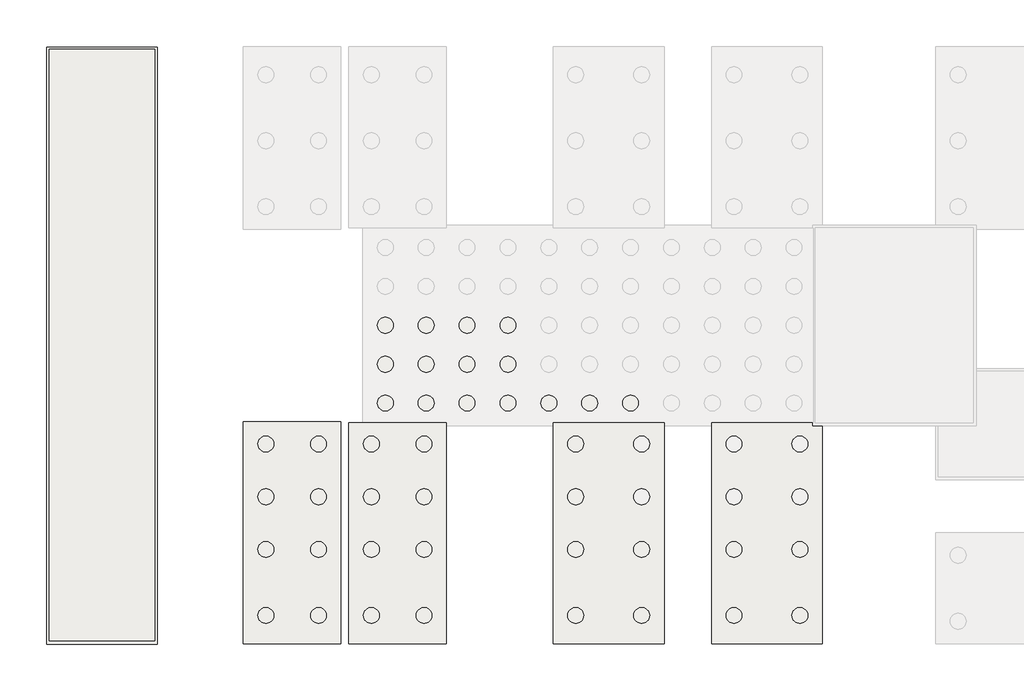
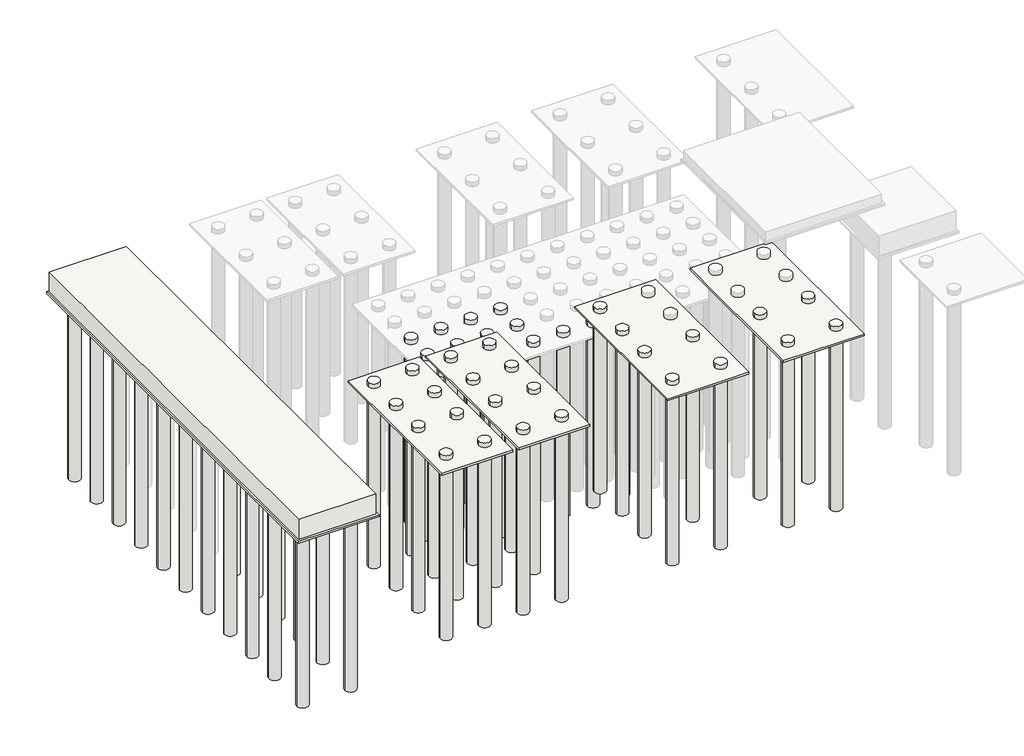
# One storey, part 1 of 3: 64 slabs.
"""IFC4 building model written with IfcOpenShell, lengths in millimetres."""

from ifc_helpers import new_model, si_unit, point, frame, frame_2d, origin, place, context, project, spatial, polyline, circle_curve, trimmed, segment, composite_curve, outline, extrude, faceted_brep, element, save

model = new_model("IFC4")

# Units and contexts
model_context = context("Model", 3, world=origin())
ifc_project = project(units=[si_unit("LENGTHUNIT", "METRE", prefix="MILLI")], contexts=[model_context])

# Site, building, storey
site = spatial("IfcSite", under=ifc_project)
building = spatial("IfcBuilding", under=site)
storey = spatial("IfcBuildingStorey", under=building, Name="B.O.F(FDN)", Elevation=-2500.0279945)

# Slabs
placement = place(None, origin())
element("IfcSlab", 1, ObjectType="H_SF_ACF_Lean_T100", at=placement, inside=storey, context=model_context, shape_type="SweptSolid", body=[
    extrude(outline(polyline([(1885.0, 41294.825326), (1885.0, 18654.825326), (-2315.0, 18654.825326), (-2315.0, 41294.825326), (1885.0, 41294.825326)])), frame((0.0, 0.0, -3699.3639791), z_axis=(0.0, 0.0, 1.0), x_axis=(1.0, 0.0, 0.0)), (0.0, 0.0, 1.0), 100.0),
])
element("IfcSlab", 2, ObjectType="H_SF_ACF_Lean_T100", at=placement, inside=storey, context=model_context, shape_type="SweptSolid", body=[
    extrude(outline(polyline([(8850.0, 27099.5208589), (8850.0, 18679.5208589), (5150.0, 18679.5208589), (5150.0, 27099.5208589), (8850.0, 27099.5208589)])), frame((0.0, 0.0, -2600.0279945), z_axis=(0.0, 0.0, 1.0), x_axis=(1.0, 0.0, 0.0)), (0.0, 0.0, 1.0), 100.0),
])
element("IfcSlab", 3, ObjectType="H_SF_ACF_Lean_T100", at=placement, inside=storey, context=model_context, shape_type="SweptSolid", body=[
    extrude(outline(polyline([(12850.0, 27049.5208589), (12850.0, 18679.5208589), (9150.0, 18679.5208589), (9150.0, 27049.5208589), (12850.0, 27049.5208589)])), frame((0.0, 0.0, -2600.0279945), z_axis=(0.0, 0.0, 1.0), x_axis=(1.0, 0.0, 0.0)), (0.0, 0.0, 1.0), 100.0),
])
element("IfcSlab", 4, ObjectType="H_SF_ACF_Lean_T100", at=placement, inside=storey, context=model_context, shape_type="SweptSolid", body=[
    extrude(outline(polyline([(21100.0, 18679.5208589), (16900.0, 18679.5208589), (16900.0, 27049.5208589), (21100.0, 27049.5208589), (21100.0, 18679.5208589)])), frame((0.0, 0.0, -2600.0279945), z_axis=(0.0, 0.0, 1.0), x_axis=(1.0, 0.0, 0.0)), (0.0, 0.0, 1.0), 100.0),
])
element("IfcSlab", 5, ObjectType="H_SF_ACF_Lean_T100", at=placement, inside=storey, context=model_context, shape_type="Brep", body=[
    faceted_brep([(27100.0, 18679.5208589, -2600.0279945), (22900.0, 18679.5208589, -2600.0279945), (22900.0, 27049.5208589, -2600.0279945), (27100.0, 27049.5208589, -2600.0279945), (27100.0, 18679.5208589, -2500.0279945), (27100.0, 27049.5208589, -2500.0279945), (26780.0, 27049.5208589, -2500.0279945), (26730.0, 27049.5208589, -2500.0279945), (22900.0, 27049.5208589, -2500.0279945), (22900.0, 18679.5208589, -2500.0279945)], [[[0, 1, 2, 3]], [[4, 5, 6, 7, 8, 9]], [[1, 0, 4, 9]], [[2, 1, 9, 8]], [[3, 2, 8, 7, 6, 5]], [[0, 3, 5, 4]]]),
])
element("IfcSlab", 6, ObjectType="Foundation Rectangular(Non-Pile) : H_SF_ACF_W4000xL22440xT1100_Protection", at=placement, inside=storey, context=model_context, shape_type="SweptSolid", body=[
    extrude(outline(polyline([(-2215.0, 41219.5208589), (1785.0, 41219.5208589), (1785.0, 18779.5208589), (-2215.0, 18779.5208589), (-2215.0, 41219.5208589)])), frame((0.0, 0.0, -3599.3639791), z_axis=(0.0, 0.0, 1.0), x_axis=(1.0, 0.0, 0.0)), (0.0, 0.0, 1.0), 1099.3359846),
])
element("IfcSlab", 7, ObjectType="Pile : H_SF_API_Steel Pile D508x12t_L10m", at=placement, inside=storey, context=model_context, shape_type="SweptSolid", body=[
    extrude(outline(composite_curve([segment(trimmed(circle_curve(frame_2d((-1465.0, 40249.5208589)), 300.0), [point((-1765.0, 40249.5208589))], [point((-1165.0, 40249.5208589))], False, "CARTESIAN"), True, "CONTINUOUS"), segment(trimmed(circle_curve(frame_2d((-1465.0, 40249.5208589)), 300.0), [point((-1165.0, 40249.5208589))], [point((-1765.0, 40249.5208589))], False, "CARTESIAN"), True, "CONTINUOUS")], self_intersect=False)), frame((0.0, 0.0, -13500.0279945), z_axis=(0.0, 0.0, 1.0), x_axis=(1.0, 0.0, 0.0)), (0.0, 0.0, 1.0), 10150.0),
])
element("IfcSlab", 8, ObjectType="Pile : H_SF_API_Steel Pile D508x12t_L10m", at=placement, inside=storey, context=model_context, shape_type="SweptSolid", body=[
    extrude(outline(composite_curve([segment(trimmed(circle_curve(frame_2d((-1465.0, 19749.5208589)), 300.0), [point((-1765.0, 19749.5208589))], [point((-1165.0, 19749.5208589))], False, "CARTESIAN"), True, "CONTINUOUS"), segment(trimmed(circle_curve(frame_2d((-1465.0, 19749.5208589)), 300.0), [point((-1165.0, 19749.5208589))], [point((-1765.0, 19749.5208589))], False, "CARTESIAN"), True, "CONTINUOUS")], self_intersect=False)), frame((0.0, 0.0, -13500.0279945), z_axis=(0.0, 0.0, 1.0), x_axis=(1.0, 0.0, 0.0)), (0.0, 0.0, 1.0), 10150.0),
])
element("IfcSlab", 9, ObjectType="Pile : H_SF_API_Steel Pile D508x12t_L10m", at=placement, inside=storey, context=model_context, shape_type="SweptSolid", body=[
    extrude(outline(composite_curve([segment(trimmed(circle_curve(frame_2d((1035.0, 19749.5208589)), 300.0), [point((1335.0, 19749.5208589))], [point((735.0, 19749.5208589))], False, "CARTESIAN"), True, "CONTINUOUS"), segment(trimmed(circle_curve(frame_2d((1035.0, 19749.5208589)), 300.0), [point((735.0, 19749.5208589))], [point((1335.0, 19749.5208589))], False, "CARTESIAN"), True, "CONTINUOUS")], self_intersect=False)), frame((0.0, 0.0, -13500.0279945), z_axis=(0.0, 0.0, 1.0), x_axis=(1.0, 0.0, 0.0)), (0.0, 0.0, 1.0), 10150.0),
])
element("IfcSlab", 10, ObjectType="Pile : H_SF_API_Steel Pile D508x12t_L10m", at=placement, inside=storey, context=model_context, shape_type="SweptSolid", body=[
    extrude(outline(composite_curve([segment(trimmed(circle_curve(frame_2d((-1465.0, 38249.5208589)), 300.0), [point((-1765.0, 38249.5208589))], [point((-1165.0, 38249.5208589))], False, "CARTESIAN"), True, "CONTINUOUS"), segment(trimmed(circle_curve(frame_2d((-1465.0, 38249.5208589)), 300.0), [point((-1165.0, 38249.5208589))], [point((-1765.0, 38249.5208589))], False, "CARTESIAN"), True, "CONTINUOUS")], self_intersect=False)), frame((0.0, 0.0, -13500.0279945), z_axis=(0.0, 0.0, 1.0), x_axis=(1.0, 0.0, 0.0)), (0.0, 0.0, 1.0), 10150.0),
])
element("IfcSlab", 11, ObjectType="Pile : H_SF_API_Steel Pile D508x12t_L10m", at=placement, inside=storey, context=model_context, shape_type="SweptSolid", body=[
    extrude(outline(composite_curve([segment(trimmed(circle_curve(frame_2d((-1465.0, 36249.5208589)), 300.0), [point((-1765.0, 36249.5208589))], [point((-1165.0, 36249.5208589))], False, "CARTESIAN"), True, "CONTINUOUS"), segment(trimmed(circle_curve(frame_2d((-1465.0, 36249.5208589)), 300.0), [point((-1165.0, 36249.5208589))], [point((-1765.0, 36249.5208589))], False, "CARTESIAN"), True, "CONTINUOUS")], self_intersect=False)), frame((0.0, 0.0, -13500.0279945), z_axis=(0.0, 0.0, 1.0), x_axis=(1.0, 0.0, 0.0)), (0.0, 0.0, 1.0), 10150.0),
])
element("IfcSlab", 12, ObjectType="Pile : H_SF_API_Steel Pile D508x12t_L10m", at=placement, inside=storey, context=model_context, shape_type="SweptSolid", body=[
    extrude(outline(composite_curve([segment(trimmed(circle_curve(frame_2d((-1465.0, 34249.5208589)), 300.0), [point((-1765.0, 34249.5208589))], [point((-1165.0, 34249.5208589))], False, "CARTESIAN"), True, "CONTINUOUS"), segment(trimmed(circle_curve(frame_2d((-1465.0, 34249.5208589)), 300.0), [point((-1165.0, 34249.5208589))], [point((-1765.0, 34249.5208589))], False, "CARTESIAN"), True, "CONTINUOUS")], self_intersect=False)), frame((0.0, 0.0, -13500.0279945), z_axis=(0.0, 0.0, 1.0), x_axis=(1.0, 0.0, 0.0)), (0.0, 0.0, 1.0), 10150.0),
])
element("IfcSlab", 13, ObjectType="Pile : H_SF_API_Steel Pile D508x12t_L10m", at=placement, inside=storey, context=model_context, shape_type="SweptSolid", body=[
    extrude(outline(composite_curve([segment(trimmed(circle_curve(frame_2d((-1465.0, 32249.5208589)), 300.0), [point((-1765.0, 32249.5208589))], [point((-1165.0, 32249.5208589))], False, "CARTESIAN"), True, "CONTINUOUS"), segment(trimmed(circle_curve(frame_2d((-1465.0, 32249.5208589)), 300.0), [point((-1165.0, 32249.5208589))], [point((-1765.0, 32249.5208589))], False, "CARTESIAN"), True, "CONTINUOUS")], self_intersect=False)), frame((0.0, 0.0, -13500.0279945), z_axis=(0.0, 0.0, 1.0), x_axis=(1.0, 0.0, 0.0)), (0.0, 0.0, 1.0), 10150.0),
])
element("IfcSlab", 14, ObjectType="Pile : H_SF_API_Steel Pile D508x12t_L10m", at=placement, inside=storey, context=model_context, shape_type="SweptSolid", body=[
    extrude(outline(composite_curve([segment(trimmed(circle_curve(frame_2d((-1465.0, 30249.5208589)), 300.0), [point((-1765.0, 30249.5208589))], [point((-1165.0, 30249.5208589))], False, "CARTESIAN"), True, "CONTINUOUS"), segment(trimmed(circle_curve(frame_2d((-1465.0, 30249.5208589)), 300.0), [point((-1165.0, 30249.5208589))], [point((-1765.0, 30249.5208589))], False, "CARTESIAN"), True, "CONTINUOUS")], self_intersect=False)), frame((0.0, 0.0, -13500.0279945), z_axis=(0.0, 0.0, 1.0), x_axis=(1.0, 0.0, 0.0)), (0.0, 0.0, 1.0), 10150.0),
])
element("IfcSlab", 15, ObjectType="Pile : H_SF_API_Steel Pile D508x12t_L10m", at=placement, inside=storey, context=model_context, shape_type="SweptSolid", body=[
    extrude(outline(composite_curve([segment(trimmed(circle_curve(frame_2d((1035.0, 30249.5208589)), 300.0), [point((1335.0, 30249.5208589))], [point((735.0, 30249.5208589))], False, "CARTESIAN"), True, "CONTINUOUS"), segment(trimmed(circle_curve(frame_2d((1035.0, 30249.5208589)), 300.0), [point((735.0, 30249.5208589))], [point((1335.0, 30249.5208589))], False, "CARTESIAN"), True, "CONTINUOUS")], self_intersect=False)), frame((0.0, 0.0, -13500.0279945), z_axis=(0.0, 0.0, 1.0), x_axis=(1.0, 0.0, 0.0)), (0.0, 0.0, 1.0), 10150.0),
])
element("IfcSlab", 16, ObjectType="Pile : H_SF_API_Steel Pile D508x12t_L10m", at=placement, inside=storey, context=model_context, shape_type="SweptSolid", body=[
    extrude(outline(composite_curve([segment(trimmed(circle_curve(frame_2d((-1465.0, 28249.5208589)), 300.0), [point((-1765.0, 28249.5208589))], [point((-1165.0, 28249.5208589))], False, "CARTESIAN"), True, "CONTINUOUS"), segment(trimmed(circle_curve(frame_2d((-1465.0, 28249.5208589)), 300.0), [point((-1165.0, 28249.5208589))], [point((-1765.0, 28249.5208589))], False, "CARTESIAN"), True, "CONTINUOUS")], self_intersect=False)), frame((0.0, 0.0, -13500.0279945), z_axis=(0.0, 0.0, 1.0), x_axis=(1.0, 0.0, 0.0)), (0.0, 0.0, 1.0), 10150.0),
])
element("IfcSlab", 17, ObjectType="Pile : H_SF_API_Steel Pile D508x12t_L10m", at=placement, inside=storey, context=model_context, shape_type="SweptSolid", body=[
    extrude(outline(composite_curve([segment(trimmed(circle_curve(frame_2d((1035.0, 28249.5208589)), 300.0), [point((1335.0, 28249.5208589))], [point((735.0, 28249.5208589))], False, "CARTESIAN"), True, "CONTINUOUS"), segment(trimmed(circle_curve(frame_2d((1035.0, 28249.5208589)), 300.0), [point((735.0, 28249.5208589))], [point((1335.0, 28249.5208589))], False, "CARTESIAN"), True, "CONTINUOUS")], self_intersect=False)), frame((0.0, 0.0, -13500.0279945), z_axis=(0.0, 0.0, 1.0), x_axis=(1.0, 0.0, 0.0)), (0.0, 0.0, 1.0), 10150.0),
])
element("IfcSlab", 18, ObjectType="Pile : H_SF_API_Steel Pile D508x12t_L10m", at=placement, inside=storey, context=model_context, shape_type="SweptSolid", body=[
    extrude(outline(composite_curve([segment(trimmed(circle_curve(frame_2d((-1465.0, 26249.5208589)), 300.0), [point((-1765.0, 26249.5208589))], [point((-1165.0, 26249.5208589))], False, "CARTESIAN"), True, "CONTINUOUS"), segment(trimmed(circle_curve(frame_2d((-1465.0, 26249.5208589)), 300.0), [point((-1165.0, 26249.5208589))], [point((-1765.0, 26249.5208589))], False, "CARTESIAN"), True, "CONTINUOUS")], self_intersect=False)), frame((0.0, 0.0, -13500.0279945), z_axis=(0.0, 0.0, 1.0), x_axis=(1.0, 0.0, 0.0)), (0.0, 0.0, 1.0), 10150.0),
])
element("IfcSlab", 19, ObjectType="Pile : H_SF_API_Steel Pile D508x12t_L10m", at=placement, inside=storey, context=model_context, shape_type="SweptSolid", body=[
    extrude(outline(composite_curve([segment(trimmed(circle_curve(frame_2d((1035.0, 26249.5208589)), 300.0), [point((1335.0, 26249.5208589))], [point((735.0, 26249.5208589))], False, "CARTESIAN"), True, "CONTINUOUS"), segment(trimmed(circle_curve(frame_2d((1035.0, 26249.5208589)), 300.0), [point((735.0, 26249.5208589))], [point((1335.0, 26249.5208589))], False, "CARTESIAN"), True, "CONTINUOUS")], self_intersect=False)), frame((0.0, 0.0, -13500.0279945), z_axis=(0.0, 0.0, 1.0), x_axis=(1.0, 0.0, 0.0)), (0.0, 0.0, 1.0), 10150.0),
])
element("IfcSlab", 20, ObjectType="Pile : H_SF_API_Steel Pile D508x12t_L10m", at=placement, inside=storey, context=model_context, shape_type="SweptSolid", body=[
    extrude(outline(composite_curve([segment(trimmed(circle_curve(frame_2d((-1465.0, 24249.5208589)), 300.0), [point((-1765.0, 24249.5208589))], [point((-1165.0, 24249.5208589))], False, "CARTESIAN"), True, "CONTINUOUS"), segment(trimmed(circle_curve(frame_2d((-1465.0, 24249.5208589)), 300.0), [point((-1165.0, 24249.5208589))], [point((-1765.0, 24249.5208589))], False, "CARTESIAN"), True, "CONTINUOUS")], self_intersect=False)), frame((0.0, 0.0, -13500.0279945), z_axis=(0.0, 0.0, 1.0), x_axis=(1.0, 0.0, 0.0)), (0.0, 0.0, 1.0), 10150.0),
])
element("IfcSlab", 21, ObjectType="Pile : H_SF_API_Steel Pile D508x12t_L10m", at=placement, inside=storey, context=model_context, shape_type="SweptSolid", body=[
    extrude(outline(composite_curve([segment(trimmed(circle_curve(frame_2d((1035.0, 24249.5208589)), 300.0), [point((1335.0, 24249.5208589))], [point((735.0, 24249.5208589))], False, "CARTESIAN"), True, "CONTINUOUS"), segment(trimmed(circle_curve(frame_2d((1035.0, 24249.5208589)), 300.0), [point((735.0, 24249.5208589))], [point((1335.0, 24249.5208589))], False, "CARTESIAN"), True, "CONTINUOUS")], self_intersect=False)), frame((0.0, 0.0, -13500.0279945), z_axis=(0.0, 0.0, 1.0), x_axis=(1.0, 0.0, 0.0)), (0.0, 0.0, 1.0), 10150.0),
])
element("IfcSlab", 22, ObjectType="Pile : H_SF_API_Steel Pile D508x12t_L10m", at=placement, inside=storey, context=model_context, shape_type="SweptSolid", body=[
    extrude(outline(composite_curve([segment(trimmed(circle_curve(frame_2d((-1465.0, 22249.5208589)), 300.0), [point((-1765.0, 22249.5208589))], [point((-1165.0, 22249.5208589))], False, "CARTESIAN"), True, "CONTINUOUS"), segment(trimmed(circle_curve(frame_2d((-1465.0, 22249.5208589)), 300.0), [point((-1165.0, 22249.5208589))], [point((-1765.0, 22249.5208589))], False, "CARTESIAN"), True, "CONTINUOUS")], self_intersect=False)), frame((0.0, 0.0, -13500.0279945), z_axis=(0.0, 0.0, 1.0), x_axis=(1.0, 0.0, 0.0)), (0.0, 0.0, 1.0), 10150.0),
])
element("IfcSlab", 23, ObjectType="Pile : H_SF_API_Steel Pile D508x12t_L10m", at=placement, inside=storey, context=model_context, shape_type="SweptSolid", body=[
    extrude(outline(composite_curve([segment(trimmed(circle_curve(frame_2d((1035.0, 22249.5208589)), 300.0), [point((1335.0, 22249.5208589))], [point((735.0, 22249.5208589))], False, "CARTESIAN"), True, "CONTINUOUS"), segment(trimmed(circle_curve(frame_2d((1035.0, 22249.5208589)), 300.0), [point((735.0, 22249.5208589))], [point((1335.0, 22249.5208589))], False, "CARTESIAN"), True, "CONTINUOUS")], self_intersect=False)), frame((0.0, 0.0, -13500.0279945), z_axis=(0.0, 0.0, 1.0), x_axis=(1.0, 0.0, 0.0)), (0.0, 0.0, 1.0), 10150.0),
])
element("IfcSlab", 24, ObjectType="Pile : H_SF_API_Steel Pile D508x12t_L10m", at=placement, inside=storey, context=model_context, shape_type="SweptSolid", body=[
    extrude(outline(composite_curve([segment(trimmed(circle_curve(frame_2d((8000.0, 19749.5208589)), 300.0), [point((8300.0, 19749.5208589))], [point((7700.0, 19749.5208589))], False, "CARTESIAN"), True, "CONTINUOUS"), segment(trimmed(circle_curve(frame_2d((8000.0, 19749.5208589)), 300.0), [point((7700.0, 19749.5208589))], [point((8300.0, 19749.5208589))], False, "CARTESIAN"), True, "CONTINUOUS")], self_intersect=False)), frame((0.0, 0.0, -12400.0279945), z_axis=(0.0, 0.0, 1.0), x_axis=(1.0, 0.0, 0.0)), (0.0, 0.0, 1.0), 10150.0),
])
element("IfcSlab", 25, ObjectType="Pile : H_SF_API_Steel Pile D508x12t_L10m", at=placement, inside=storey, context=model_context, shape_type="SweptSolid", body=[
    extrude(outline(composite_curve([segment(trimmed(circle_curve(frame_2d((6000.0, 19749.5208589)), 300.0), [point((5700.0, 19749.5208589))], [point((6300.0, 19749.5208589))], False, "CARTESIAN"), True, "CONTINUOUS"), segment(trimmed(circle_curve(frame_2d((6000.0, 19749.5208589)), 300.0), [point((6300.0, 19749.5208589))], [point((5700.0, 19749.5208589))], False, "CARTESIAN"), True, "CONTINUOUS")], self_intersect=False)), frame((0.0, 0.0, -12400.0279945), z_axis=(0.0, 0.0, 1.0), x_axis=(1.0, 0.0, 0.0)), (0.0, 0.0, 1.0), 10150.0),
])
element("IfcSlab", 26, ObjectType="Pile : H_SF_API_Steel Pile D508x12t_L10m", at=placement, inside=storey, context=model_context, shape_type="SweptSolid", body=[
    extrude(outline(composite_curve([segment(trimmed(circle_curve(frame_2d((8000.0, 22249.5208589)), 300.0), [point((8300.0, 22249.5208589))], [point((7700.0, 22249.5208589))], False, "CARTESIAN"), True, "CONTINUOUS"), segment(trimmed(circle_curve(frame_2d((8000.0, 22249.5208589)), 300.0), [point((7700.0, 22249.5208589))], [point((8300.0, 22249.5208589))], False, "CARTESIAN"), True, "CONTINUOUS")], self_intersect=False)), frame((0.0, 0.0, -12400.0279945), z_axis=(0.0, 0.0, 1.0), x_axis=(1.0, 0.0, 0.0)), (0.0, 0.0, 1.0), 10150.0),
])
element("IfcSlab", 27, ObjectType="Pile : H_SF_API_Steel Pile D508x12t_L10m", at=placement, inside=storey, context=model_context, shape_type="SweptSolid", body=[
    extrude(outline(composite_curve([segment(trimmed(circle_curve(frame_2d((6000.0, 22249.5208589)), 300.0), [point((5700.0, 22249.5208589))], [point((6300.0, 22249.5208589))], False, "CARTESIAN"), True, "CONTINUOUS"), segment(trimmed(circle_curve(frame_2d((6000.0, 22249.5208589)), 300.0), [point((6300.0, 22249.5208589))], [point((5700.0, 22249.5208589))], False, "CARTESIAN"), True, "CONTINUOUS")], self_intersect=False)), frame((0.0, 0.0, -12400.0279945), z_axis=(0.0, 0.0, 1.0), x_axis=(1.0, 0.0, 0.0)), (0.0, 0.0, 1.0), 10150.0),
])
element("IfcSlab", 28, ObjectType="Pile : H_SF_API_Steel Pile D508x12t_L10m", at=placement, inside=storey, context=model_context, shape_type="SweptSolid", body=[
    extrude(outline(composite_curve([segment(trimmed(circle_curve(frame_2d((8000.0, 24249.5208589)), 300.0), [point((8300.0, 24249.5208589))], [point((7700.0, 24249.5208589))], False, "CARTESIAN"), True, "CONTINUOUS"), segment(trimmed(circle_curve(frame_2d((8000.0, 24249.5208589)), 300.0), [point((7700.0, 24249.5208589))], [point((8300.0, 24249.5208589))], False, "CARTESIAN"), True, "CONTINUOUS")], self_intersect=False)), frame((0.0, 0.0, -12400.0279945), z_axis=(0.0, 0.0, 1.0), x_axis=(1.0, 0.0, 0.0)), (0.0, 0.0, 1.0), 10150.0),
])
element("IfcSlab", 29, ObjectType="Pile : H_SF_API_Steel Pile D508x12t_L10m", at=placement, inside=storey, context=model_context, shape_type="SweptSolid", body=[
    extrude(outline(composite_curve([segment(trimmed(circle_curve(frame_2d((6000.0, 24249.5208589)), 300.0), [point((5700.0, 24249.5208589))], [point((6300.0, 24249.5208589))], False, "CARTESIAN"), True, "CONTINUOUS"), segment(trimmed(circle_curve(frame_2d((6000.0, 24249.5208589)), 300.0), [point((6300.0, 24249.5208589))], [point((5700.0, 24249.5208589))], False, "CARTESIAN"), True, "CONTINUOUS")], self_intersect=False)), frame((0.0, 0.0, -12400.0279945), z_axis=(0.0, 0.0, 1.0), x_axis=(1.0, 0.0, 0.0)), (0.0, 0.0, 1.0), 10150.0),
])
element("IfcSlab", 30, ObjectType="Pile : H_SF_API_Steel Pile D508x12t_L10m", at=placement, inside=storey, context=model_context, shape_type="SweptSolid", body=[
    extrude(outline(composite_curve([segment(trimmed(circle_curve(frame_2d((8000.0, 26249.5208589)), 300.0), [point((8300.0, 26249.5208589))], [point((7700.0, 26249.5208589))], False, "CARTESIAN"), True, "CONTINUOUS"), segment(trimmed(circle_curve(frame_2d((8000.0, 26249.5208589)), 300.0), [point((7700.0, 26249.5208589))], [point((8300.0, 26249.5208589))], False, "CARTESIAN"), True, "CONTINUOUS")], self_intersect=False)), frame((0.0, 0.0, -12400.0279945), z_axis=(0.0, 0.0, 1.0), x_axis=(1.0, 0.0, 0.0)), (0.0, 0.0, 1.0), 10150.0),
])
element("IfcSlab", 31, ObjectType="Pile : H_SF_API_Steel Pile D508x12t_L10m", at=placement, inside=storey, context=model_context, shape_type="SweptSolid", body=[
    extrude(outline(composite_curve([segment(trimmed(circle_curve(frame_2d((6000.0, 26249.5208589)), 300.0), [point((5700.0, 26249.5208589))], [point((6300.0, 26249.5208589))], False, "CARTESIAN"), True, "CONTINUOUS"), segment(trimmed(circle_curve(frame_2d((6000.0, 26249.5208589)), 300.0), [point((6300.0, 26249.5208589))], [point((5700.0, 26249.5208589))], False, "CARTESIAN"), True, "CONTINUOUS")], self_intersect=False)), frame((0.0, 0.0, -12400.0279945), z_axis=(0.0, 0.0, 1.0), x_axis=(1.0, 0.0, 0.0)), (0.0, 0.0, 1.0), 10150.0),
])
element("IfcSlab", 32, ObjectType="Pile : H_SF_API_Steel Pile D508x12t_L10m", at=placement, inside=storey, context=model_context, shape_type="SweptSolid", body=[
    extrude(outline(composite_curve([segment(trimmed(circle_curve(frame_2d((12000.0, 19749.5208589)), 300.0), [point((12300.0, 19749.5208589))], [point((11700.0, 19749.5208589))], False, "CARTESIAN"), True, "CONTINUOUS"), segment(trimmed(circle_curve(frame_2d((12000.0, 19749.5208589)), 300.0), [point((11700.0, 19749.5208589))], [point((12300.0, 19749.5208589))], False, "CARTESIAN"), True, "CONTINUOUS")], self_intersect=False)), frame((0.0, 0.0, -12400.0279945), z_axis=(0.0, 0.0, 1.0), x_axis=(1.0, 0.0, 0.0)), (0.0, 0.0, 1.0), 10150.0),
])
element("IfcSlab", 33, ObjectType="Pile : H_SF_API_Steel Pile D508x12t_L10m", at=placement, inside=storey, context=model_context, shape_type="SweptSolid", body=[
    extrude(outline(composite_curve([segment(trimmed(circle_curve(frame_2d((10000.0, 19749.5208589)), 300.0), [point((9700.0, 19749.5208589))], [point((10300.0, 19749.5208589))], False, "CARTESIAN"), True, "CONTINUOUS"), segment(trimmed(circle_curve(frame_2d((10000.0, 19749.5208589)), 300.0), [point((10300.0, 19749.5208589))], [point((9700.0, 19749.5208589))], False, "CARTESIAN"), True, "CONTINUOUS")], self_intersect=False)), frame((0.0, 0.0, -12400.0279945), z_axis=(0.0, 0.0, 1.0), x_axis=(1.0, 0.0, 0.0)), (0.0, 0.0, 1.0), 10150.0),
])
element("IfcSlab", 34, ObjectType="Pile : H_SF_API_Steel Pile D508x12t_L10m", at=placement, inside=storey, context=model_context, shape_type="SweptSolid", body=[
    extrude(outline(composite_curve([segment(trimmed(circle_curve(frame_2d((12000.0, 22249.5208589)), 300.0), [point((12300.0, 22249.5208589))], [point((11700.0, 22249.5208589))], False, "CARTESIAN"), True, "CONTINUOUS"), segment(trimmed(circle_curve(frame_2d((12000.0, 22249.5208589)), 300.0), [point((11700.0, 22249.5208589))], [point((12300.0, 22249.5208589))], False, "CARTESIAN"), True, "CONTINUOUS")], self_intersect=False)), frame((0.0, 0.0, -12400.0279945), z_axis=(0.0, 0.0, 1.0), x_axis=(1.0, 0.0, 0.0)), (0.0, 0.0, 1.0), 10150.0),
])
element("IfcSlab", 35, ObjectType="Pile : H_SF_API_Steel Pile D508x12t_L10m", at=placement, inside=storey, context=model_context, shape_type="SweptSolid", body=[
    extrude(outline(composite_curve([segment(trimmed(circle_curve(frame_2d((10000.0, 22249.5208589)), 300.0), [point((9700.0, 22249.5208589))], [point((10300.0, 22249.5208589))], False, "CARTESIAN"), True, "CONTINUOUS"), segment(trimmed(circle_curve(frame_2d((10000.0, 22249.5208589)), 300.0), [point((10300.0, 22249.5208589))], [point((9700.0, 22249.5208589))], False, "CARTESIAN"), True, "CONTINUOUS")], self_intersect=False)), frame((0.0, 0.0, -12400.0279945), z_axis=(0.0, 0.0, 1.0), x_axis=(1.0, 0.0, 0.0)), (0.0, 0.0, 1.0), 10150.0),
])
element("IfcSlab", 36, ObjectType="Pile : H_SF_API_Steel Pile D508x12t_L10m", at=placement, inside=storey, context=model_context, shape_type="SweptSolid", body=[
    extrude(outline(composite_curve([segment(trimmed(circle_curve(frame_2d((12000.0, 24249.5208589)), 300.0), [point((12300.0, 24249.5208589))], [point((11700.0, 24249.5208589))], False, "CARTESIAN"), True, "CONTINUOUS"), segment(trimmed(circle_curve(frame_2d((12000.0, 24249.5208589)), 300.0), [point((11700.0, 24249.5208589))], [point((12300.0, 24249.5208589))], False, "CARTESIAN"), True, "CONTINUOUS")], self_intersect=False)), frame((0.0, 0.0, -12400.0279945), z_axis=(0.0, 0.0, 1.0), x_axis=(1.0, 0.0, 0.0)), (0.0, 0.0, 1.0), 10150.0),
])
element("IfcSlab", 37, ObjectType="Pile : H_SF_API_Steel Pile D508x12t_L10m", at=placement, inside=storey, context=model_context, shape_type="SweptSolid", body=[
    extrude(outline(composite_curve([segment(trimmed(circle_curve(frame_2d((10000.0, 24249.5208589)), 300.0), [point((9700.0, 24249.5208589))], [point((10300.0, 24249.5208589))], False, "CARTESIAN"), True, "CONTINUOUS"), segment(trimmed(circle_curve(frame_2d((10000.0, 24249.5208589)), 300.0), [point((10300.0, 24249.5208589))], [point((9700.0, 24249.5208589))], False, "CARTESIAN"), True, "CONTINUOUS")], self_intersect=False)), frame((0.0, 0.0, -12400.0279945), z_axis=(0.0, 0.0, 1.0), x_axis=(1.0, 0.0, 0.0)), (0.0, 0.0, 1.0), 10150.0),
])
element("IfcSlab", 38, ObjectType="Pile : H_SF_API_Steel Pile D508x12t_L10m", at=placement, inside=storey, context=model_context, shape_type="SweptSolid", body=[
    extrude(outline(composite_curve([segment(trimmed(circle_curve(frame_2d((12000.0, 26249.5208589)), 300.0), [point((12300.0, 26249.5208589))], [point((11700.0, 26249.5208589))], False, "CARTESIAN"), True, "CONTINUOUS"), segment(trimmed(circle_curve(frame_2d((12000.0, 26249.5208589)), 300.0), [point((11700.0, 26249.5208589))], [point((12300.0, 26249.5208589))], False, "CARTESIAN"), True, "CONTINUOUS")], self_intersect=False)), frame((0.0, 0.0, -12400.0279945), z_axis=(0.0, 0.0, 1.0), x_axis=(1.0, 0.0, 0.0)), (0.0, 0.0, 1.0), 10150.0),
])
element("IfcSlab", 39, ObjectType="Pile : H_SF_API_Steel Pile D508x12t_L10m", at=placement, inside=storey, context=model_context, shape_type="SweptSolid", body=[
    extrude(outline(composite_curve([segment(trimmed(circle_curve(frame_2d((10000.0, 26249.5208589)), 300.0), [point((9700.0, 26249.5208589))], [point((10300.0, 26249.5208589))], False, "CARTESIAN"), True, "CONTINUOUS"), segment(trimmed(circle_curve(frame_2d((10000.0, 26249.5208589)), 300.0), [point((10300.0, 26249.5208589))], [point((9700.0, 26249.5208589))], False, "CARTESIAN"), True, "CONTINUOUS")], self_intersect=False)), frame((0.0, 0.0, -12400.0279945), z_axis=(0.0, 0.0, 1.0), x_axis=(1.0, 0.0, 0.0)), (0.0, 0.0, 1.0), 10150.0),
])
element("IfcSlab", 40, ObjectType="Pile : H_SF_API_Steel Pile D508x12t_L10m", at=placement, inside=storey, context=model_context, shape_type="SweptSolid", body=[
    extrude(outline(composite_curve([segment(trimmed(circle_curve(frame_2d((20250.0, 19749.5208589)), 300.0), [point((20550.0, 19749.5208589))], [point((19950.0, 19749.5208589))], False, "CARTESIAN"), True, "CONTINUOUS"), segment(trimmed(circle_curve(frame_2d((20250.0, 19749.5208589)), 300.0), [point((19950.0, 19749.5208589))], [point((20550.0, 19749.5208589))], False, "CARTESIAN"), True, "CONTINUOUS")], self_intersect=False)), frame((0.0, 0.0, -12400.0279945), z_axis=(0.0, 0.0, 1.0), x_axis=(1.0, 0.0, 0.0)), (0.0, 0.0, 1.0), 10150.0),
])
element("IfcSlab", 41, ObjectType="Pile : H_SF_API_Steel Pile D508x12t_L10m", at=placement, inside=storey, context=model_context, shape_type="SweptSolid", body=[
    extrude(outline(composite_curve([segment(trimmed(circle_curve(frame_2d((17750.0, 19749.5208589)), 300.0), [point((17450.0, 19749.5208589))], [point((18050.0, 19749.5208589))], False, "CARTESIAN"), True, "CONTINUOUS"), segment(trimmed(circle_curve(frame_2d((17750.0, 19749.5208589)), 300.0), [point((18050.0, 19749.5208589))], [point((17450.0, 19749.5208589))], False, "CARTESIAN"), True, "CONTINUOUS")], self_intersect=False)), frame((0.0, 0.0, -12400.0279945), z_axis=(0.0, 0.0, 1.0), x_axis=(1.0, 0.0, 0.0)), (0.0, 0.0, 1.0), 10150.0),
])
element("IfcSlab", 42, ObjectType="Pile : H_SF_API_Steel Pile D508x12t_L10m", at=placement, inside=storey, context=model_context, shape_type="SweptSolid", body=[
    extrude(outline(composite_curve([segment(trimmed(circle_curve(frame_2d((20250.0, 22249.5208589)), 300.0), [point((20550.0, 22249.5208589))], [point((19950.0, 22249.5208589))], False, "CARTESIAN"), True, "CONTINUOUS"), segment(trimmed(circle_curve(frame_2d((20250.0, 22249.5208589)), 300.0), [point((19950.0, 22249.5208589))], [point((20550.0, 22249.5208589))], False, "CARTESIAN"), True, "CONTINUOUS")], self_intersect=False)), frame((0.0, 0.0, -12400.0279945), z_axis=(0.0, 0.0, 1.0), x_axis=(1.0, 0.0, 0.0)), (0.0, 0.0, 1.0), 10150.0),
])
element("IfcSlab", 43, ObjectType="Pile : H_SF_API_Steel Pile D508x12t_L10m", at=placement, inside=storey, context=model_context, shape_type="SweptSolid", body=[
    extrude(outline(composite_curve([segment(trimmed(circle_curve(frame_2d((17750.0, 22249.5208589)), 300.0), [point((17450.0, 22249.5208589))], [point((18050.0, 22249.5208589))], False, "CARTESIAN"), True, "CONTINUOUS"), segment(trimmed(circle_curve(frame_2d((17750.0, 22249.5208589)), 300.0), [point((18050.0, 22249.5208589))], [point((17450.0, 22249.5208589))], False, "CARTESIAN"), True, "CONTINUOUS")], self_intersect=False)), frame((0.0, 0.0, -12400.0279945), z_axis=(0.0, 0.0, 1.0), x_axis=(1.0, 0.0, 0.0)), (0.0, 0.0, 1.0), 10150.0),
])
element("IfcSlab", 44, ObjectType="Pile : H_SF_API_Steel Pile D508x12t_L10m", at=placement, inside=storey, context=model_context, shape_type="SweptSolid", body=[
    extrude(outline(composite_curve([segment(trimmed(circle_curve(frame_2d((17750.0, 24249.5208589)), 300.0), [point((17450.0, 24249.5208589))], [point((18050.0, 24249.5208589))], False, "CARTESIAN"), True, "CONTINUOUS"), segment(trimmed(circle_curve(frame_2d((17750.0, 24249.5208589)), 300.0), [point((18050.0, 24249.5208589))], [point((17450.0, 24249.5208589))], False, "CARTESIAN"), True, "CONTINUOUS")], self_intersect=False)), frame((0.0, 0.0, -12400.0279945), z_axis=(0.0, 0.0, 1.0), x_axis=(1.0, 0.0, 0.0)), (0.0, 0.0, 1.0), 10150.0),
])
element("IfcSlab", 45, ObjectType="Pile : H_SF_API_Steel Pile D508x12t_L10m", at=placement, inside=storey, context=model_context, shape_type="SweptSolid", body=[
    extrude(outline(composite_curve([segment(trimmed(circle_curve(frame_2d((17750.0, 26249.5208589)), 300.0), [point((17450.0, 26249.5208589))], [point((18050.0, 26249.5208589))], False, "CARTESIAN"), True, "CONTINUOUS"), segment(trimmed(circle_curve(frame_2d((17750.0, 26249.5208589)), 300.0), [point((18050.0, 26249.5208589))], [point((17450.0, 26249.5208589))], False, "CARTESIAN"), True, "CONTINUOUS")], self_intersect=False)), frame((0.0, 0.0, -12400.0279945), z_axis=(0.0, 0.0, 1.0), x_axis=(1.0, 0.0, 0.0)), (0.0, 0.0, 1.0), 10150.0),
])
element("IfcSlab", 46, ObjectType="Pile : H_SF_API_Steel Pile D508x12t_L10m", at=placement, inside=storey, context=model_context, shape_type="SweptSolid", body=[
    extrude(outline(composite_curve([segment(trimmed(circle_curve(frame_2d((26250.0, 19749.5208589)), 300.0), [point((26550.0, 19749.5208589))], [point((25950.0, 19749.5208589))], False, "CARTESIAN"), True, "CONTINUOUS"), segment(trimmed(circle_curve(frame_2d((26250.0, 19749.5208589)), 300.0), [point((25950.0, 19749.5208589))], [point((26550.0, 19749.5208589))], False, "CARTESIAN"), True, "CONTINUOUS")], self_intersect=False)), frame((0.0, 0.0, -12400.0279945), z_axis=(0.0, 0.0, 1.0), x_axis=(1.0, 0.0, 0.0)), (0.0, 0.0, 1.0), 10150.0),
])
element("IfcSlab", 47, ObjectType="Pile : H_SF_API_Steel Pile D508x12t_L10m", at=placement, inside=storey, context=model_context, shape_type="SweptSolid", body=[
    extrude(outline(composite_curve([segment(trimmed(circle_curve(frame_2d((23750.0, 19749.5208589)), 300.0), [point((23450.0, 19749.5208589))], [point((24050.0, 19749.5208589))], False, "CARTESIAN"), True, "CONTINUOUS"), segment(trimmed(circle_curve(frame_2d((23750.0, 19749.5208589)), 300.0), [point((24050.0, 19749.5208589))], [point((23450.0, 19749.5208589))], False, "CARTESIAN"), True, "CONTINUOUS")], self_intersect=False)), frame((0.0, 0.0, -12400.0279945), z_axis=(0.0, 0.0, 1.0), x_axis=(1.0, 0.0, 0.0)), (0.0, 0.0, 1.0), 10150.0),
])
element("IfcSlab", 48, ObjectType="Pile : H_SF_API_Steel Pile D508x12t_L10m", at=placement, inside=storey, context=model_context, shape_type="SweptSolid", body=[
    extrude(outline(composite_curve([segment(trimmed(circle_curve(frame_2d((26250.0, 22249.5208589)), 300.0), [point((26550.0, 22249.5208589))], [point((25950.0, 22249.5208589))], False, "CARTESIAN"), True, "CONTINUOUS"), segment(trimmed(circle_curve(frame_2d((26250.0, 22249.5208589)), 300.0), [point((25950.0, 22249.5208589))], [point((26550.0, 22249.5208589))], False, "CARTESIAN"), True, "CONTINUOUS")], self_intersect=False)), frame((0.0, 0.0, -12400.0279945), z_axis=(0.0, 0.0, 1.0), x_axis=(1.0, 0.0, 0.0)), (0.0, 0.0, 1.0), 10150.0),
])
element("IfcSlab", 49, ObjectType="Pile : H_SF_API_Steel Pile D508x12t_L10m", at=placement, inside=storey, context=model_context, shape_type="SweptSolid", body=[
    extrude(outline(composite_curve([segment(trimmed(circle_curve(frame_2d((23750.0, 22249.5208589)), 300.0), [point((23450.0, 22249.5208589))], [point((24050.0, 22249.5208589))], False, "CARTESIAN"), True, "CONTINUOUS"), segment(trimmed(circle_curve(frame_2d((23750.0, 22249.5208589)), 300.0), [point((24050.0, 22249.5208589))], [point((23450.0, 22249.5208589))], False, "CARTESIAN"), True, "CONTINUOUS")], self_intersect=False)), frame((0.0, 0.0, -12400.0279945), z_axis=(0.0, 0.0, 1.0), x_axis=(1.0, 0.0, 0.0)), (0.0, 0.0, 1.0), 10150.0),
])
element("IfcSlab", 50, ObjectType="Pile : H_SF_API_Steel Pile D508x12t_L10m", at=placement, inside=storey, context=model_context, shape_type="SweptSolid", body=[
    extrude(outline(composite_curve([segment(trimmed(circle_curve(frame_2d((10530.0, 27799.5208589)), 300.0), [point((10230.0, 27799.5208589))], [point((10830.0, 27799.5208589))], False, "CARTESIAN"), True, "CONTINUOUS"), segment(trimmed(circle_curve(frame_2d((10530.0, 27799.5208589)), 300.0), [point((10830.0, 27799.5208589))], [point((10230.0, 27799.5208589))], False, "CARTESIAN"), True, "CONTINUOUS")], self_intersect=False)), frame((0.0, 0.0, -14300.0279945), z_axis=(0.0, 0.0, 1.0), x_axis=(1.0, 0.0, 0.0)), (0.0, 0.0, 1.0), 10150.0),
])
element("IfcSlab", 51, ObjectType="Pile : H_SF_API_Steel Pile D508x12t_L10m", at=placement, inside=storey, context=model_context, shape_type="SweptSolid", body=[
    extrude(outline(composite_curve([segment(trimmed(circle_curve(frame_2d((10530.0, 29274.5208589)), 300.0), [point((10230.0, 29274.5208589))], [point((10830.0, 29274.5208589))], False, "CARTESIAN"), True, "CONTINUOUS"), segment(trimmed(circle_curve(frame_2d((10530.0, 29274.5208589)), 300.0), [point((10830.0, 29274.5208589))], [point((10230.0, 29274.5208589))], False, "CARTESIAN"), True, "CONTINUOUS")], self_intersect=False)), frame((0.0, 0.0, -14300.0279945), z_axis=(0.0, 0.0, 1.0), x_axis=(1.0, 0.0, 0.0)), (0.0, 0.0, 1.0), 10150.0),
])
element("IfcSlab", 52, ObjectType="Pile : H_SF_API_Steel Pile D508x12t_L10m", at=placement, inside=storey, context=model_context, shape_type="SweptSolid", body=[
    extrude(outline(composite_curve([segment(trimmed(circle_curve(frame_2d((10530.0, 30749.5208589)), 300.0), [point((10230.0, 30749.5208589))], [point((10830.0, 30749.5208589))], False, "CARTESIAN"), True, "CONTINUOUS"), segment(trimmed(circle_curve(frame_2d((10530.0, 30749.5208589)), 300.0), [point((10830.0, 30749.5208589))], [point((10230.0, 30749.5208589))], False, "CARTESIAN"), True, "CONTINUOUS")], self_intersect=False)), frame((0.0, 0.0, -14300.0279945), z_axis=(0.0, 0.0, 1.0), x_axis=(1.0, 0.0, 0.0)), (0.0, 0.0, 1.0), 10150.0),
])
element("IfcSlab", 53, ObjectType="Pile : H_SF_API_Steel Pile D508x12t_L10m", at=placement, inside=storey, context=model_context, shape_type="SweptSolid", body=[
    extrude(outline(composite_curve([segment(trimmed(circle_curve(frame_2d((19830.0, 27799.5208589)), 300.0), [point((20130.0, 27799.5208589))], [point((19530.0, 27799.5208589))], False, "CARTESIAN"), True, "CONTINUOUS"), segment(trimmed(circle_curve(frame_2d((19830.0, 27799.5208589)), 300.0), [point((19530.0, 27799.5208589))], [point((20130.0, 27799.5208589))], False, "CARTESIAN"), True, "CONTINUOUS")], self_intersect=False)), frame((0.0, 0.0, -14300.0279945), z_axis=(0.0, 0.0, 1.0), x_axis=(1.0, 0.0, 0.0)), (0.0, 0.0, 1.0), 10150.0),
])
element("IfcSlab", 54, ObjectType="Pile : H_SF_API_Steel Pile D508x12t_L10m", at=placement, inside=storey, context=model_context, shape_type="SweptSolid", body=[
    extrude(outline(composite_curve([segment(trimmed(circle_curve(frame_2d((18280.0, 27799.5208589)), 300.0), [point((18580.0, 27799.5208589))], [point((17980.0, 27799.5208589))], False, "CARTESIAN"), True, "CONTINUOUS"), segment(trimmed(circle_curve(frame_2d((18280.0, 27799.5208589)), 300.0), [point((17980.0, 27799.5208589))], [point((18580.0, 27799.5208589))], False, "CARTESIAN"), True, "CONTINUOUS")], self_intersect=False)), frame((0.0, 0.0, -14300.0279945), z_axis=(0.0, 0.0, 1.0), x_axis=(1.0, 0.0, 0.0)), (0.0, 0.0, 1.0), 10150.0),
])
element("IfcSlab", 55, ObjectType="Pile : H_SF_API_Steel Pile D508x12t_L10m", at=placement, inside=storey, context=model_context, shape_type="SweptSolid", body=[
    extrude(outline(composite_curve([segment(trimmed(circle_curve(frame_2d((16730.0, 27799.5208589)), 300.0), [point((17030.0, 27799.5208589))], [point((16430.0, 27799.5208589))], False, "CARTESIAN"), True, "CONTINUOUS"), segment(trimmed(circle_curve(frame_2d((16730.0, 27799.5208589)), 300.0), [point((16430.0, 27799.5208589))], [point((17030.0, 27799.5208589))], False, "CARTESIAN"), True, "CONTINUOUS")], self_intersect=False)), frame((0.0, 0.0, -14300.0279945), z_axis=(0.0, 0.0, 1.0), x_axis=(1.0, 0.0, 0.0)), (0.0, 0.0, 1.0), 10150.0),
])
element("IfcSlab", 56, ObjectType="Pile : H_SF_API_Steel Pile D508x12t_L10m", at=placement, inside=storey, context=model_context, shape_type="SweptSolid", body=[
    extrude(outline(composite_curve([segment(trimmed(circle_curve(frame_2d((15180.0, 27799.5208589)), 300.0), [point((15480.0, 27799.5208589))], [point((14880.0, 27799.5208589))], False, "CARTESIAN"), True, "CONTINUOUS"), segment(trimmed(circle_curve(frame_2d((15180.0, 27799.5208589)), 300.0), [point((14880.0, 27799.5208589))], [point((15480.0, 27799.5208589))], False, "CARTESIAN"), True, "CONTINUOUS")], self_intersect=False)), frame((0.0, 0.0, -14300.0279945), z_axis=(0.0, 0.0, 1.0), x_axis=(1.0, 0.0, 0.0)), (0.0, 0.0, 1.0), 10150.0),
])
element("IfcSlab", 57, ObjectType="Pile : H_SF_API_Steel Pile D508x12t_L10m", at=placement, inside=storey, context=model_context, shape_type="SweptSolid", body=[
    extrude(outline(composite_curve([segment(trimmed(circle_curve(frame_2d((15180.0, 29274.5208589)), 300.0), [point((15480.0, 29274.5208589))], [point((14880.0, 29274.5208589))], False, "CARTESIAN"), True, "CONTINUOUS"), segment(trimmed(circle_curve(frame_2d((15180.0, 29274.5208589)), 300.0), [point((14880.0, 29274.5208589))], [point((15480.0, 29274.5208589))], False, "CARTESIAN"), True, "CONTINUOUS")], self_intersect=False)), frame((0.0, 0.0, -14300.0279945), z_axis=(0.0, 0.0, 1.0), x_axis=(1.0, 0.0, 0.0)), (0.0, 0.0, 1.0), 10150.0),
])
element("IfcSlab", 58, ObjectType="Pile : H_SF_API_Steel Pile D508x12t_L10m", at=placement, inside=storey, context=model_context, shape_type="SweptSolid", body=[
    extrude(outline(composite_curve([segment(trimmed(circle_curve(frame_2d((15180.0, 30749.5208589)), 300.0), [point((15480.0, 30749.5208589))], [point((14880.0, 30749.5208589))], False, "CARTESIAN"), True, "CONTINUOUS"), segment(trimmed(circle_curve(frame_2d((15180.0, 30749.5208589)), 300.0), [point((14880.0, 30749.5208589))], [point((15480.0, 30749.5208589))], False, "CARTESIAN"), True, "CONTINUOUS")], self_intersect=False)), frame((0.0, 0.0, -14300.0279945), z_axis=(0.0, 0.0, 1.0), x_axis=(1.0, 0.0, 0.0)), (0.0, 0.0, 1.0), 10150.0),
])
element("IfcSlab", 59, ObjectType="Pile : H_SF_API_Steel Pile D508x12t_L10m", at=placement, inside=storey, context=model_context, shape_type="SweptSolid", body=[
    extrude(outline(composite_curve([segment(trimmed(circle_curve(frame_2d((13630.0, 27799.5208589)), 300.0), [point((13930.0, 27799.5208589))], [point((13330.0, 27799.5208589))], False, "CARTESIAN"), True, "CONTINUOUS"), segment(trimmed(circle_curve(frame_2d((13630.0, 27799.5208589)), 300.0), [point((13330.0, 27799.5208589))], [point((13930.0, 27799.5208589))], False, "CARTESIAN"), True, "CONTINUOUS")], self_intersect=False)), frame((0.0, 0.0, -14300.0279945), z_axis=(0.0, 0.0, 1.0), x_axis=(1.0, 0.0, 0.0)), (0.0, 0.0, 1.0), 10150.0),
])
element("IfcSlab", 60, ObjectType="Pile : H_SF_API_Steel Pile D508x12t_L10m", at=placement, inside=storey, context=model_context, shape_type="SweptSolid", body=[
    extrude(outline(composite_curve([segment(trimmed(circle_curve(frame_2d((13630.0, 29274.5208589)), 300.0), [point((13930.0, 29274.5208589))], [point((13330.0, 29274.5208589))], False, "CARTESIAN"), True, "CONTINUOUS"), segment(trimmed(circle_curve(frame_2d((13630.0, 29274.5208589)), 300.0), [point((13330.0, 29274.5208589))], [point((13930.0, 29274.5208589))], False, "CARTESIAN"), True, "CONTINUOUS")], self_intersect=False)), frame((0.0, 0.0, -14300.0279945), z_axis=(0.0, 0.0, 1.0), x_axis=(1.0, 0.0, 0.0)), (0.0, 0.0, 1.0), 10150.0),
])
element("IfcSlab", 61, ObjectType="Pile : H_SF_API_Steel Pile D508x12t_L10m", at=placement, inside=storey, context=model_context, shape_type="SweptSolid", body=[
    extrude(outline(composite_curve([segment(trimmed(circle_curve(frame_2d((13630.0, 30749.5208589)), 300.0), [point((13930.0, 30749.5208589))], [point((13330.0, 30749.5208589))], False, "CARTESIAN"), True, "CONTINUOUS"), segment(trimmed(circle_curve(frame_2d((13630.0, 30749.5208589)), 300.0), [point((13330.0, 30749.5208589))], [point((13930.0, 30749.5208589))], False, "CARTESIAN"), True, "CONTINUOUS")], self_intersect=False)), frame((0.0, 0.0, -14300.0279945), z_axis=(0.0, 0.0, 1.0), x_axis=(1.0, 0.0, 0.0)), (0.0, 0.0, 1.0), 10150.0),
])
element("IfcSlab", 62, ObjectType="Pile : H_SF_API_Steel Pile D508x12t_L10m", at=placement, inside=storey, context=model_context, shape_type="SweptSolid", body=[
    extrude(outline(composite_curve([segment(trimmed(circle_curve(frame_2d((12080.0, 27799.5208589)), 300.0), [point((12380.0, 27799.5208589))], [point((11780.0, 27799.5208589))], False, "CARTESIAN"), True, "CONTINUOUS"), segment(trimmed(circle_curve(frame_2d((12080.0, 27799.5208589)), 300.0), [point((11780.0, 27799.5208589))], [point((12380.0, 27799.5208589))], False, "CARTESIAN"), True, "CONTINUOUS")], self_intersect=False)), frame((0.0, 0.0, -14300.0279945), z_axis=(0.0, 0.0, 1.0), x_axis=(1.0, 0.0, 0.0)), (0.0, 0.0, 1.0), 10150.0),
])
element("IfcSlab", 63, ObjectType="Pile : H_SF_API_Steel Pile D508x12t_L10m", at=placement, inside=storey, context=model_context, shape_type="SweptSolid", body=[
    extrude(outline(composite_curve([segment(trimmed(circle_curve(frame_2d((12080.0, 29274.5208589)), 300.0), [point((12380.0, 29274.5208589))], [point((11780.0, 29274.5208589))], False, "CARTESIAN"), True, "CONTINUOUS"), segment(trimmed(circle_curve(frame_2d((12080.0, 29274.5208589)), 300.0), [point((11780.0, 29274.5208589))], [point((12380.0, 29274.5208589))], False, "CARTESIAN"), True, "CONTINUOUS")], self_intersect=False)), frame((0.0, 0.0, -14300.0279945), z_axis=(0.0, 0.0, 1.0), x_axis=(1.0, 0.0, 0.0)), (0.0, 0.0, 1.0), 10150.0),
])
element("IfcSlab", 64, ObjectType="Pile : H_SF_API_Steel Pile D508x12t_L10m", at=placement, inside=storey, context=model_context, shape_type="SweptSolid", body=[
    extrude(outline(composite_curve([segment(trimmed(circle_curve(frame_2d((12080.0, 30749.5208589)), 300.0), [point((12380.0, 30749.5208589))], [point((11780.0, 30749.5208589))], False, "CARTESIAN"), True, "CONTINUOUS"), segment(trimmed(circle_curve(frame_2d((12080.0, 30749.5208589)), 300.0), [point((11780.0, 30749.5208589))], [point((12380.0, 30749.5208589))], False, "CARTESIAN"), True, "CONTINUOUS")], self_intersect=False)), frame((0.0, 0.0, -14300.0279945), z_axis=(0.0, 0.0, 1.0), x_axis=(1.0, 0.0, 0.0)), (0.0, 0.0, 1.0), 10150.0),
])

save(model, "model.ifc")

# Revit data of these elements
# Project information
#   Building Name = "STEAM TURBINE BUILDING"
#   H_Building Tag = "STB"
#   Project Status = "종결"
#   Client Name = "Therma Viayas Inc.\nTherma Viayas Inc.\nTherma Viayas Inc.\nTherma Viayas Inc."
#   Project Name = "Therma Visayas 2*150MW CFB Power Plant"
#   Project Number = "BEPH1402"
# Grids (mm)
#   "1": line (0, 42917.66) -> (0, 17977.903)
#   "5": line (25000, 42917.66) -> (25000, 17977.903)
#   "6": line (33500, 42917.66) -> (33500, 17977.903)
#   "7": line (40000, 42917.66) -> (40000, 17977.903)
#   "A": line (-3740.747, 20999.521) -> (54382.977, 20999.521)
#   "B": line (-3740.747, 26999.521) -> (54382.977, 26999.521)
#   "C": line (-3740.747, 32999.521) -> (54382.977, 32999.521)
#   "D": line (-3740.747, 38999.521) -> (54382.977, 38999.521)
#   "2": line (7000, 42917.66) -> (7000, 17977.903)
#   "3": line (11000, 42917.66) -> (11000, 17977.903)
#   "4": line (19000, 42917.66) -> (19000, 17977.903)
#   "8": line (50000, 42917.66) -> (50000, 17977.903)
# Type "H_SF_ACF_Lean_T100"
#   Type Comments = "구조_콘크리트"
#   H_WM Code_1 = "A03AD034-00004 | Concrete Work | Substructure Work | Lean Concrete (including Form work) | Cement Type-1 | 10MPa < F'c (Cylinder Strength) ≤ 20MPa"
#   H_WM Code_2 = "A01ZZ005-00001 | Earth Work | - | Base Course | THK≤150mm | THK=(  )mm | CBR=(  )%"
#   H_WM Code_3 = "A01ZZ006-00001 | Earth Work | - | Subbase Course | Including Compaction of Sub-Grade | THK≤150mm | THK=(  )mm | CBR=(  )% for Subgrade, (  )% for Subbase | Compaction=(  )% for Subgrade, (  )% for Subbase"
#   H_WM Code_4 = "A01ZZ012-00001 | Earth Work | - | PE Sheet (Vapor Barrier) | THK=(  )mm"
#   H_Q'ty Cal Type Tag = "SF-Q3"
#   Layers, outside or top first: 0.1000 m "A03AC034-00004_Lean Concrete (including Form work)" (function 1)
# Type "Foundation Rectangular(Non-Pile) : H_SF_ACF_W4000xL22440xT1100_Protection"
#   H_WM Code_1 = "A03AD032-00012 | Concrete Work | Substructure Work | Structural Concrete | Cement Type-5 | 20MPa < F'c (Cylinder Strength) ≤ 25MPa"
#   H_WM Code_2 = "A03AD037-00002 | Concrete Work | Substructure Work | Rebar Work | Deformed Bar (Non-Coat.) | 400MPa<Fy≤470MPa"
#   H_WM Code_3 = "A03AD035-00001 | Concrete Work | Substructure Work | Form Work (3 times in use) | Flat Form | Dressed Lumber, Plywood or Steel Form(Wood Planks are not Allowed) incl. Chamfer"
#   H_WM Code_4 = "A03AH056-00001 | Concrete Work | Concrete Protective Coating (U/G) | Bitumen/Bituminous/Asphalt Coating"
#   H_WM Code_5 = "A03AH059-00001 | Concrete Work | Concrete Protective Coating (U/G) | Sheet Membrane | Adhesive Rubber Sheet or Bitumen Polyethylene Laminated Waterproofing Membrane | THK=(  )mm"
#   H_WM Code_6 = "A03AH060-00001 | Concrete Work | Concrete Protective Coating (U/G) | Memebrane Protection Board | Bitumen Impregnated Fiberboard | THK=(  )mm"
#   H_WM Code_7 = "A01ZZ001-00005 | Earth Work | - | Excavation | Soil, Mech. | 2.0M < D ≤ 4.0M"
#   H_WM Code_8 = "A01ZZ003-00001 | Earth Work | - | Backfill | Re-use, Soil | Compaction=(  )%"
#   H_WM Code_9 = "A01ZZ004-00001 | Earth Work | - | Disposal | Soil | Disposal Distance=Appx. (  )km from Site"
#   H_Q'ty Cal Type Tag = "SF-Q4"
#   Top bar = "D25@300"
#   Description = "UG Shallow Foundation"
#   Bottom bar = "D20@300"
#   Width = 4.0000 m
#   Length = 22.4400 m
#   Foundation Thickness = 1.1000 m
#   Structural Material [instance default] = A03AD032-00010_Structural Concrete_UG_20-24MPa
#   Assembly Code = ""
# Type "Pile : H_SF_API_Steel Pile D508x12t_L10m"
#   Type Mark = ""
#   H_WM Code_1 = "A02AA020-00001 | Pile Work | Piling Work | Steel Pipe Pile Work | Direct Driving | Including Pile Connection and Joint Welding Work | D=(  )mm / THK=(  )mm | Pile Length per Hole=(  )M"
#   H_WM Code_2 = "A02AB020-00001 | Pile Work | Pile Head Treatment | Steel Pipe Pile Work | D=(  )mm / THK=(  )mm"
#   H_Q'ty Cal Type Tag = "SF-Q5"
#   Assembly Code = "A1020130"
#   반지름 = 0.3000 m
#   최소 내포 = 0.1500 m
#   Diameter = 0.6000 m
#   Depth = 10.0000 m
#   VISIBLE [instance default] = yes
#   구조 재료 = 콘크리트
# Element 1 (IfcSlab, "H_SF_ACF_Lean_T100")
#   Comments = ""
#   Height Offset From Level = -1.099336 m
#   built-in parameter 1001954 = 1
#   Phase Created = New Construction
#   Materials on its faces: "A03AC034-00004_Lean Concrete (including Form work)"
# Elements 2, 3, 4, 5 (IfcSlab, "H_SF_ACF_Lean_T100")
#   Comments = ""
#   Height Offset From Level = 0.0000 m
#   built-in parameter 1001954 = 1
#   Phase Created = New Construction
#   Materials on its faces: "A03AC034-00004_Lean Concrete (including Form work)"
# Element 6 (IfcSlab, "Foundation Rectangular(Non-Pile) : H_SF_ACF_W4000xL22440xT1100_Protection")
#   Comments = ""
#   Mark = "F1"
#   Structural Material = A03AD032-00010_Structural Concrete_UG_20-24MPa
#   Phase Created = New Construction
#   Materials on its faces: "A03AD032-00010_Structural Concrete_UG_20-24MPa"
# Element 7 (IfcSlab, "Pile : H_SF_API_Steel Pile D508x12t_L10m")
#   Mark = "P101"
#   Phase Created = New Construction
#   Materials on its faces: "금속 - 스틸 - 345MPa"
# Elements 8, 9, 12, 13, 14, 15, 16, 17, 18, 19, 20, 21, 22, 23, 25, 26, 27, 28, 29, 30, 31, 32, 33, 34, 35, 36, 37, 38, 39, 40, 41, 42, 43, 44, 45, 47, 49, 50, 51, 52, 53, 54, 55, 56, 57, 58, 59, 60, 61, 62, 63, 64 (IfcSlab, "Pile : H_SF_API_Steel Pile D508x12t_L10m")
#   Phase Created = New Construction
#   Materials on its faces: "금속 - 스틸 - 345MPa"
# Element 10 (IfcSlab, "Pile : H_SF_API_Steel Pile D508x12t_L10m")
#   Mark = "103"
#   Phase Created = New Construction
#   Materials on its faces: "금속 - 스틸 - 345MPa"
# Element 11 (IfcSlab, "Pile : H_SF_API_Steel Pile D508x12t_L10m")
#   Mark = "105"
#   Phase Created = New Construction
#   Materials on its faces: "금속 - 스틸 - 345MPa"
# Element 24 (IfcSlab, "Pile : H_SF_API_Steel Pile D508x12t_L10m")
#   Mark = "P123"
#   Phase Created = New Construction
#   Materials on its faces: "금속 - 스틸 - 345MPa"
# Elements 46, 48 (IfcSlab, "Pile : H_SF_API_Steel Pile D508x12t_L10m")
#   VISIBLE = yes
#   Phase Created = New Construction
#   Materials on its faces: "금속 - 스틸 - 345MPa"
# Materials
#   "A03AC034-00004_Lean Concrete (including Form work)": class "Concrete", colour RGB 176 176 176, transparency 0, Description = "Plain Conc.", Cost = 0
#   "A03AD032-00010_Structural Concrete_UG_20-24MPa": class "Concrete", colour RGB 176 176 176, transparency 0, Keynote = "09910.A1", Description = "Substructure Concrete / Cement Type-1 / 24MPa", Cost = 0
#   "콘크리트": class "*D 철근콘크리트공사", colour RGB 192 192 192, transparency 0, Keynote = "DF", Description = "콘크리트", Cost = 0
#   "금속 - 스틸 - 345MPa": class "금속", colour RGB 247 247 247, transparency 0
